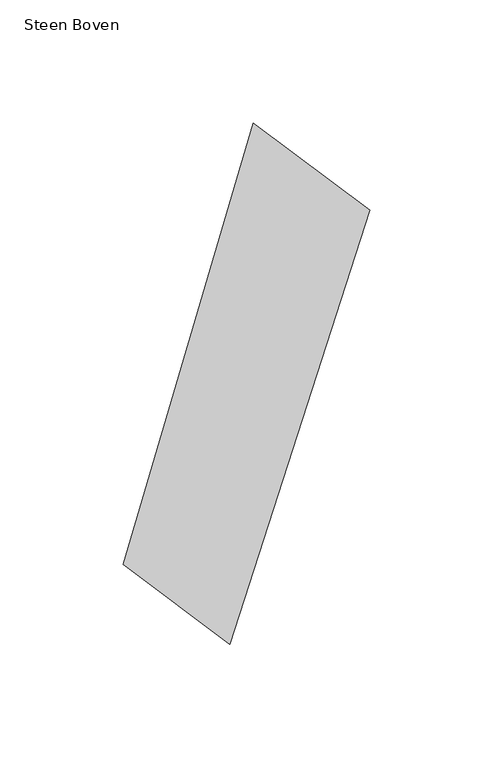
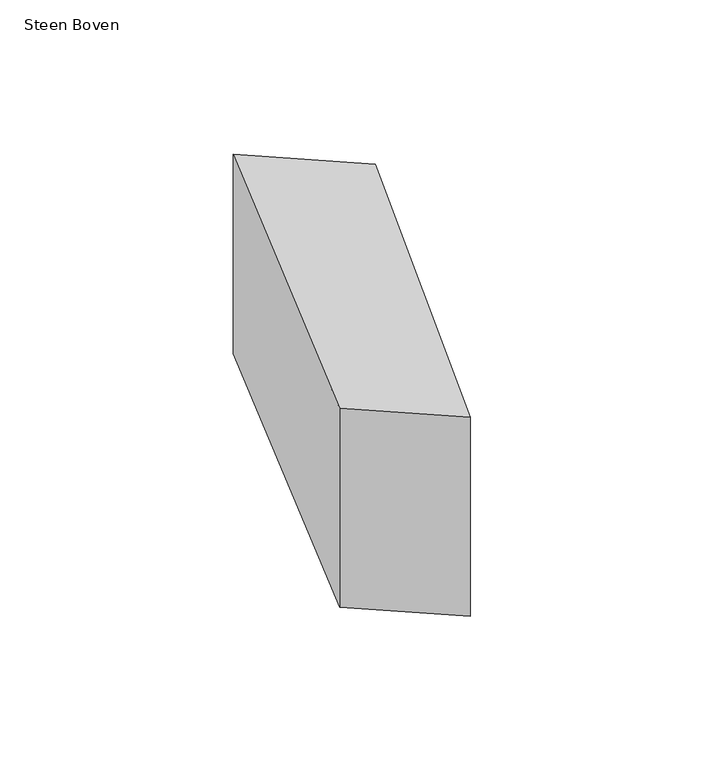
"""IFC4 building model written with IfcOpenShell, lengths in millimetres: proxy geometry, 00_GMA_steen_versie_4 : Steen Boven."""

import ifcopenshell
import ifcopenshell.guid

model = None  # the IFC model being written
_history = None  # IfcOwnerHistory: only IFC2X3 demands one
_inside = {}  # id of a spatial element -> (the spatial element, [elements in it])
_under = {}  # id of a project, library or spatial element -> (it, [spatial elements below it])
_declared = {}  # id of a project -> (the project, [libraries it declares])
_typed = {}  # id of a type object -> (the type object, [elements of that type])
_made_of = {}  # id of a material, layer set ... -> (it, [elements and type objects made of it])


def new_model(schema):
    """Start an empty IFC model of exactly this schema.

    Asked for "IFC4X3", IfcOpenShell would pick the latest addendum, in which some entities
    have other attributes; the version numbers below select the first issue.
    IFC2X3 requires an IfcOwnerHistory on every rooted entity: one is made here for all.
    """
    global model, _history
    if schema == "IFC4X3":
        model = ifcopenshell.file(schema_version=(4, 3, 0, 0))
    else:
        model = ifcopenshell.file(schema=schema)
    _inside.clear()
    _under.clear()
    _declared.clear()
    _typed.clear()
    _made_of.clear()
    _history = None
    if model.schema == "IFC2X3":
        org = make("IfcOrganization", Name="unknown")
        user = make(
            "IfcPersonAndOrganization",
            ThePerson=make("IfcPerson", FamilyName="unknown"),
            TheOrganization=org,
        )
        app = make(
            "IfcApplication",
            ApplicationDeveloper=org,
            Version="unknown",
            ApplicationFullName="unknown",
            ApplicationIdentifier="unknown",
        )
        _history = make(
            "IfcOwnerHistory",
            OwningUser=user,
            OwningApplication=app,
            ChangeAction="ADDED",
            CreationDate=0,
        )
    return model


def make(cls, **values):
    """One entity of the class cls with the attributes given. An attribute that is None is left unset."""
    return model.create_entity(
        cls, **{name: value for name, value in values.items() if value is not None}
    )


def rooted(cls, **values):
    """An entity with a GlobalId (a new one), such as an element, a storey or a relation."""
    return make(cls, GlobalId=ifcopenshell.guid.new(), OwnerHistory=_history, **values)


def si_unit(unit_type, name, prefix=None):
    """IfcSIUnit, for example si_unit("LENGTHUNIT", "METRE", prefix="MILLI")."""
    return make("IfcSIUnit", UnitType=unit_type, Prefix=prefix, Name=name)


def assignment(units):
    """IfcUnitAssignment: the units of a project."""
    return None if units is None else make("IfcUnitAssignment", Units=units)


def point(xyz):
    """IfcCartesianPoint."""
    return None if xyz is None else make("IfcCartesianPoint", Coordinates=xyz)


def direction(xyz):
    """IfcDirection."""
    return None if xyz is None else make("IfcDirection", DirectionRatios=xyz)


def frame(location, z_axis=None, x_axis=None):
    """IfcAxis2Placement3D, a coordinate frame: its origin and axes. An axis left out is left unset."""
    return make(
        "IfcAxis2Placement3D",
        Location=point(location),
        Axis=direction(z_axis),
        RefDirection=direction(x_axis),
    )


def origin():
    """The frame at (0, 0, 0) with its axes left unset."""
    return frame((0.0, 0.0, 0.0))


def origin_with_axes():
    """The frame at (0, 0, 0) with the z axis (0, 0, 1) and the x axis (1, 0, 0) written out."""
    return frame((0.0, 0.0, 0.0), z_axis=(0.0, 0.0, 1.0), x_axis=(1.0, 0.0, 0.0))


def place(relative_to, where):
    """IfcLocalPlacement: puts the frame where relative to a parent placement (None: the world)."""
    return make(
        "IfcLocalPlacement", PlacementRelTo=relative_to, RelativePlacement=where
    )


def context(
    kind, dimensions, precision=None, world=None, true_north=None, identifier=None
):
    """IfcGeometricRepresentationContext, for example the 3D "Model" context."""
    return make(
        "IfcGeometricRepresentationContext",
        ContextIdentifier=identifier,
        ContextType=kind,
        CoordinateSpaceDimension=dimensions,
        Precision=precision,
        WorldCoordinateSystem=world,
        TrueNorth=true_north,
    )


def project(units=None, contexts=None):
    """IfcProject with its units and contexts."""
    return rooted(
        "IfcProject",
        Name="project",
        RepresentationContexts=contexts,
        UnitsInContext=assignment(units),
    )


def spatial(cls, under=None, at=None, **own):
    """A site, building, storey or space (cls), placed at a placement, below another one or the project."""
    s = rooted(cls, ObjectPlacement=at, **own)
    if under is not None:
        _under.setdefault(under.id(), (under, []))[1].append(s)
    return s


def polyline(points):
    """IfcPolyline through the points."""
    return make("IfcPolyline", Points=[point(p) for p in points])


def outline(outer, holes=None, kind="AREA"):
    """IfcArbitraryClosedProfileDef: a profile drawn as a closed curve; with holes, ...WithVoids."""
    if holes is None:
        return make("IfcArbitraryClosedProfileDef", ProfileType=kind, OuterCurve=outer)
    return make(
        "IfcArbitraryProfileDefWithVoids",
        ProfileType=kind,
        OuterCurve=outer,
        InnerCurves=holes,
    )


def extrude(swept, where, along, depth):
    """IfcExtrudedAreaSolid: the profile swept, set in the frame where, extruded along a direction by depth."""
    return make(
        "IfcExtrudedAreaSolid",
        SweptArea=swept,
        Position=where,
        ExtrudedDirection=direction(along),
        Depth=depth,
    )


def shape(context_of_items, identifier, shape_type, items):
    """IfcShapeRepresentation: the items that make up one representation, for example the "Body"."""
    return make(
        "IfcShapeRepresentation",
        ContextOfItems=context_of_items,
        RepresentationIdentifier=identifier,
        RepresentationType=shape_type,
        Items=items,
    )


def source(mapping_origin, context_of_items, identifier, shape_type, items):
    """IfcRepresentationMap: a shape defined once, which mapped items show again and again."""
    return make(
        "IfcRepresentationMap",
        MappingOrigin=mapping_origin,
        MappedRepresentation=shape(context_of_items, identifier, shape_type, items),
    )


def transform(
    local_origin,
    x_axis=None,
    y_axis=None,
    z_axis=None,
    scale=None,
    scale2=None,
    scale3=None,
    uniform=True,
):
    """IfcCartesianTransformationOperator3D, or its non-uniform kind. x_axis, y_axis, z_axis: its Axis1, 2, 3."""
    if uniform:
        return make(
            "IfcCartesianTransformationOperator3D",
            Axis1=direction(x_axis),
            Axis2=direction(y_axis),
            LocalOrigin=point(local_origin),
            Scale=scale,
            Axis3=direction(z_axis),
        )
    return make(
        "IfcCartesianTransformationOperator3DnonUniform",
        Axis1=direction(x_axis),
        Axis2=direction(y_axis),
        LocalOrigin=point(local_origin),
        Scale=scale,
        Axis3=direction(z_axis),
        Scale2=scale2,
        Scale3=scale3,
    )


def mapped(mapping_source, mapping_target):
    """IfcMappedItem: shows the shape of a source again, moved by a transform."""
    return make(
        "IfcMappedItem", MappingSource=mapping_source, MappingTarget=mapping_target
    )


def made_of(thing, what):
    """Note that an element or type object is made of a material, layer set ...; save() writes the relation."""
    if what is not None:
        _made_of.setdefault(what.id(), (what, []))[1].append(thing)
    return thing


def element(
    cls,
    number,
    at=None,
    inside=None,
    cuts=None,
    type_object=None,
    material=None,
    context=None,
    identifier="Body",
    shape_type=None,
    held_by="IfcProductDefinitionShape",
    body=None,
    shapes=None,
    **own,
):
    """One element of the class cls, such as IfcWall. Its Tag is "e" and its number.

    at: its placement. inside: the storey or other place that contains it. cuts: it is an
    opening in that element (IfcRelVoidsElement). A single representation is given by context,
    identifier, shape_type and body (its items); several are given by shapes. held_by: the class
    of the entity that holds the representations. save() writes the other relations.
    """
    e = rooted(cls, Tag="e%d" % number, ObjectPlacement=at, **own)
    if body is not None:
        shapes = [shape(context, identifier, shape_type, body)]
    if shapes is not None:
        e.Representation = make(held_by, Representations=shapes)
    if inside is not None:
        _inside.setdefault(inside.id(), (inside, []))[1].append(e)
    if cuts is not None:
        rooted(
            "IfcRelVoidsElement", RelatingBuildingElement=cuts, RelatedOpeningElement=e
        )
    if type_object is not None:
        _typed.setdefault(type_object.id(), (type_object, []))[1].append(e)
    return made_of(e, material)


def aggregate(whole, parts):
    """IfcRelAggregates: a whole, such as a stair, and the parts it consists of."""
    return rooted("IfcRelAggregates", RelatingObject=whole, RelatedObjects=parts)


def save(model, path):
    """Write the relations noted so far, then the file.

    IfcRelAggregates (storeys below a building ...), IfcRelContainedInSpatialStructure (elements
    in a storey), IfcRelDefinesByType, IfcRelAssociatesMaterial and IfcRelDeclares: one each for
    every whole, place, type object, material and project.
    """
    for whole, parts in _under.values():
        aggregate(whole, parts)
    for where, things in _inside.values():
        rooted(
            "IfcRelContainedInSpatialStructure",
            RelatedElements=things,
            RelatingStructure=where,
        )
    for kind, things in _typed.values():
        rooted("IfcRelDefinesByType", RelatedObjects=things, RelatingType=kind)
    for what, things in _made_of.values():
        rooted("IfcRelAssociatesMaterial", RelatedObjects=things, RelatingMaterial=what)
    for by, libraries in _declared.values():
        rooted("IfcRelDeclares", RelatingContext=by, RelatedDefinitions=libraries)
    model.write(path)


def steen_boven_663f693a(model_context):
    return source(origin(), model_context, "Body", "SweptSolid", [
        extrude(outline(polyline([(130.7162887, 162.2194761), (73.9191357, -14.270629), (30.6030106, 18.1662603), (83.5403775, 197.5941228), (130.7162887, 162.2194761)])), origin_with_axes(), (0.0, 0.0, 1.0), 100.0),
    ])


if __name__ == "__main__":
    model = new_model("IFC4")
    model_context = context("Model", 3, world=origin())
    ifc_project = project(units=[si_unit("LENGTHUNIT", "METRE", prefix="MILLI")], contexts=[model_context])
    site = spatial("IfcSite", under=ifc_project)
    building = spatial("IfcBuilding", under=site)
    placement = place(None, origin())
    steen_boven_shape = steen_boven_663f693a(model_context)
    element("IfcBuildingElementProxy", 1, Name="00_GMA_steen_versie_4 : Steen Boven", ObjectType="00_GMA_steen_versie_4 : Steen Boven", at=placement, inside=building, context=model_context, shape_type="MappedRepresentation", body=[
        mapped(steen_boven_shape, transform((0.0, 0.0, 0.0), x_axis=(1.0, 0.0, 0.0), y_axis=(0.0, 1.0, 0.0), z_axis=(0.0, 0.0, 1.0))),
    ])
    save(model, "model.ifc")

# Revit data of these elements
# Type "00_GMA_steen_versie_4 : Steen Boven"
#   StootVoegHalfBoven [instance default] = 5 mm
#   StootVoegHalf [instance default] = 5 mm
#   StootVoegBreedteOnder = 10 mm
#   StootVoegBreedteBoven = 10 mm
#   Steendikte = 100 mm
#   LintVoegOnderHalf = 5 mm
#   LintVoegOnder = 10 mm
#   LintVoegBovenHalf = 0 mm
#   LintVoegBoven = 0 mm
#   materiaal = none
#   MateriaalVoeg = none
#   Default Elevation = 0
